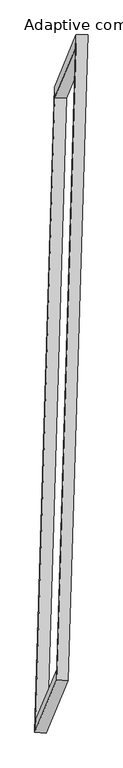
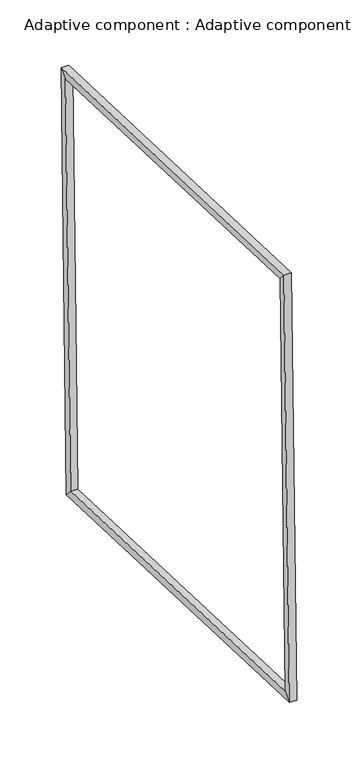
"""IFC4 building model written with IfcOpenShell, lengths in millimetres: proxy geometry, Adaptive component : Adaptive component."""

from ifc_helpers import new_model, si_unit, origin, place, context, project, spatial, faceted_brep, source, transform, mapped, element, save


def adaptive_component_adaptive_component_29a1ac7c(model_context):
    return source(origin(), model_context, "Body", "Brep", [
        faceted_brep([(94.6319235, 1535.9789681, 3098.7341305), (159.6571744, 1535.818766, 3098.4803404), (36.6377116, 1241.9680639, -693.8834929), (-28.2687994, 1242.4118944, -689.9692651), (92.391601, 1466.1568863, 3039.0140794), (-26.3085649, 1182.6234822, -620.19728), (157.4168519, 1465.9966842, 3038.7602893), (38.5979461, 1182.1796517, -624.1115077), (-73.7973948, -2378.5287116, -409.7675076), (-138.5922542, -2374.4245025, -406.1405255), (-132.6822201, -2304.7229656, -346.5301748), (-67.8873607, -2308.8271747, -350.1571569), (49.2220681, -2084.6780095, 3382.5963256), (-15.6915313, -2080.8574288, 3382.5628701), (-13.9820543, -2021.1895615, 3312.6811846), (50.931545, -2025.0101423, 3312.7146402)], [[[0, 1, 2, 3]], [[4, 0, 3, 5]], [[6, 4, 5, 7]], [[1, 6, 7, 2]], [[3, 2, 8, 9]], [[5, 3, 9, 10]], [[7, 5, 10, 11]], [[2, 7, 11, 8]], [[9, 8, 12, 13]], [[10, 9, 13, 14]], [[11, 10, 14, 15]], [[8, 11, 15, 12]], [[13, 12, 1, 0]], [[14, 13, 0, 4]], [[15, 14, 4, 6]], [[12, 15, 6, 1]]]),
    ])


if __name__ == "__main__":
    model = new_model("IFC4")
    model_context = context("Model", 3, world=origin())
    ifc_project = project(units=[si_unit("LENGTHUNIT", "METRE", prefix="MILLI")], contexts=[model_context])
    site = spatial("IfcSite", under=ifc_project)
    building = spatial("IfcBuilding", under=site)
    placement = place(None, origin())
    adaptive_component_adaptive_component_shape = adaptive_component_adaptive_component_29a1ac7c(model_context)
    element("IfcBuildingElementProxy", 1, Name="Adaptive component : Adaptive component", ObjectType="Adaptive component : Adaptive component", at=placement, inside=building, context=model_context, shape_type="MappedRepresentation", body=[
        mapped(adaptive_component_adaptive_component_shape, transform((0.0, 0.0, 0.0), x_axis=(1.0, 0.0, 0.0), y_axis=(0.0, 1.0, 0.0), z_axis=(0.0, 0.0, 1.0))),
    ])
    save(model, "model.ifc")

# Revit data of these elements
# Type "Adaptive component : Adaptive component"
#   r [instance default] = 2063.125 mm
#   2r [instance default] = 4126.251 mm
#   Number [instance default] = 5
#   Default Elevation = 0
# Element 1 (IfcBuildingElementProxy, "Adaptive component : Adaptive component")
#   r = 2536.564 mm
#   2r = 5073.128 mm
#   Number = 22
